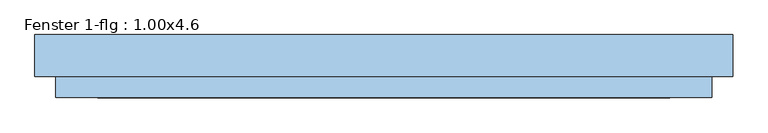
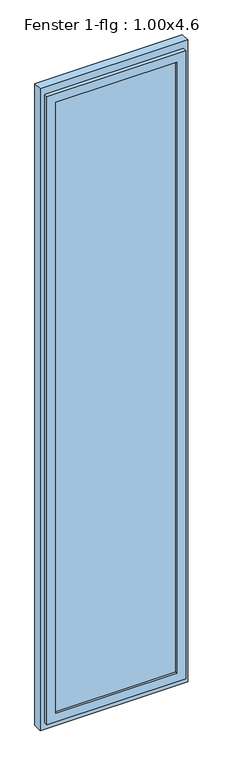
"""IFC4 building model written with IfcOpenShell, lengths in millimetres: window geometry, Fenster 1-flg : 1.00x4.6."""

from ifc_helpers import new_model, si_unit, frame, origin, place, context, project, spatial, polyline, outline, extrude, faceted_brep, source, transform, mapped, element, save


def fenster_1_flg_1_00x4_6_654662e2(model_context):
    return source(origin(), model_context, "Body", "SolidModel", [
        extrude(outline(polyline([(5600.0, 500.0), (5600.0, -500.0), (1000.0, -500.0), (1000.0, 500.0), (5600.0, 500.0)]), holes=[polyline([(5520.0, 440.0), (1080.0, 440.0), (1080.0, -440.0), (5520.0, -440.0), (5520.0, 440.0)])]), frame((0.0, -15.0, 0.0), z_axis=(0.0, 1.0, 0.0), x_axis=(0.0, 0.0, 1.0)), (0.0, 0.0, 1.0), 60.0),
        faceted_brep([(470.0, -15.0, 5550.0), (470.0, -45.0, 5550.0), (470.0, -45.0, 1050.0), (470.0, -15.0, 1050.0), (-470.0, -45.0, 5550.0), (-470.0, -45.0, 1050.0), (410.0, -45.0, 1110.0), (-410.0, -45.0, 1110.0), (-410.0, -45.0, 5490.0), (410.0, -45.0, 5490.0), (-470.0, -15.0, 1050.0), (-470.0, -15.0, 5550.0), (440.0, -15.0, 5520.0), (-440.0, -15.0, 5520.0), (-440.0, -15.0, 1080.0), (440.0, -15.0, 1080.0), (440.0, 15.0, 5520.0), (440.0, 15.0, 1080.0), (-440.0, 15.0, 1080.0), (-440.0, 15.0, 5520.0), (410.0, 15.0, 5490.0), (-410.0, 15.0, 5490.0), (-410.0, 15.0, 1110.0), (410.0, 15.0, 1110.0)], [[[0, 1, 2, 3]], [[1, 4, 5, 2], [6, 7, 8, 9]], [[3, 2, 5, 10]], [[3, 10, 11, 0], [12, 13, 14, 15]], [[16, 12, 15, 17]], [[17, 15, 14, 18]], [[17, 18, 19, 16], [20, 21, 22, 23]], [[9, 20, 23, 6]], [[6, 23, 22, 7]], [[10, 5, 4, 11]], [[18, 14, 13, 19]], [[7, 22, 21, 8]], [[11, 4, 1, 0]], [[19, 13, 12, 16]], [[8, 21, 20, 9]]]),
        extrude(outline(polyline([(410.0, -30.0), (-410.0, -30.0), (-410.0, 0.0), (410.0, 0.0), (410.0, -30.0)])), frame((0.0, 0.0, 1110.0), z_axis=(0.0, 0.0, 1.0), x_axis=(1.0, 0.0, 0.0)), (0.0, 0.0, 1.0), 4380.0),
    ])


if __name__ == "__main__":
    model = new_model("IFC4")
    model_context = context("Model", 3, world=origin())
    ifc_project = project(units=[si_unit("LENGTHUNIT", "METRE", prefix="MILLI")], contexts=[model_context])
    site = spatial("IfcSite", under=ifc_project)
    building = spatial("IfcBuilding", under=site)
    placement = place(None, origin())
    fenster_1_flg_1_00x4_6_shape = fenster_1_flg_1_00x4_6_654662e2(model_context)
    element("IfcWindow", 1, ObjectType="Fenster 1-flg : 1.00x4.6", at=placement, inside=building, context=model_context, shape_type="MappedRepresentation", body=[
        mapped(fenster_1_flg_1_00x4_6_shape, transform((0.0, 0.0, 0.0), x_axis=(1.0, 0.0, 0.0), y_axis=(0.0, 1.0, 0.0), z_axis=(0.0, 0.0, 1.0))),
    ])
    save(model, "model.ifc")

# Revit data of these elements
# Type "Fenster 1-flg : 1.00x4.6"
#   Type Mark = "78"
#   Operation = "SinglePanel"
#   Keynote = "16.05.01"
#   Visual Light Transmittance = 0.9
#   Solar Heat Gain Coefficient = 0.86
#   Rough Width = 1.000 m
#   Rough Height = 4.600 m
#   Heat Transfer Coefficient (U) = 5.5617 W/(m²·K)
#   Rahmentiefe = 0.060 m
#   Rahmenhöhe - unten = 0.080 m
#   Rahmenhöhe - oben = 0.080 m
#   Rahmenbreite = 0.060 m
#   Height = 4.600 m
#   Tiefe Flügel = 0.060 m
#   Flügelbreite = 0.060 m
#   Einbautiefe (von außen) [instance default] = 0.100 m
#   Width = 1.000 m
#   Klappflügel [instance default] = no
#   Kippflügel [instance default] = yes
#   Öffnungsrichtung in Draufsicht anzeigen [instance default] = no
#   Drehflügel 1 [instance default] = yes
#   Rahmen 1 [instance default] = none
#   Glas [instance default] = none
#   Flügel [instance default] = none
#   Fensterbank Innenseite [instance default] = none
#   Fensterbank Außenseite [instance default] = none
#   Construction Type Id = ""
#   Wall Closure = (empty or 0)
#   Analytic Construction = (empty or 0)
# Element 1 (IfcWindow, "Fenster 1-flg : 1.00x4.6")
#   Einbautiefe (von außen) = 0.230 m
#   Materials on its faces: "Kunststoff - Weiß", "Glas"
# Materials
#   "Kunststoff - Weiß": class "Kunststoff", colour RGB 249 249 249, transparency 0, Cost = 0
#   "Glas": class "Glas", colour RGB 0 0 255, transparency 0.75, Comments = "Render-Darstellung nicht aktualisiert ", Cost = 0
